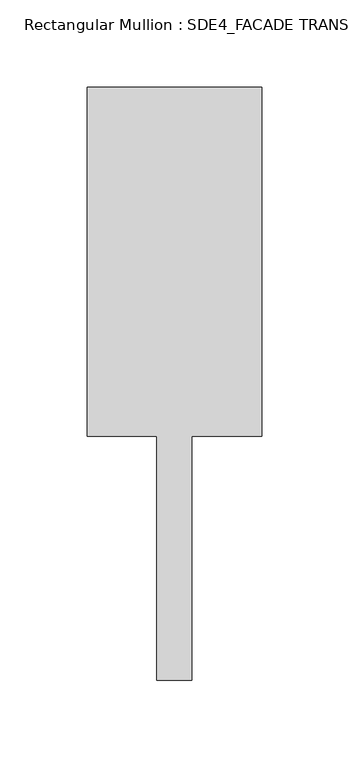
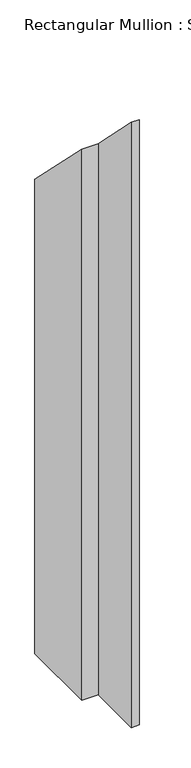
"""IFC4 building model written with IfcOpenShell, lengths in millimetres: member geometry, Rectangular Mullion : SDE4_FACADE TRANSOM TYPE 1."""

from ifc_helpers import new_model, si_unit, origin, place, context, project, spatial, faceted_brep, source, transform, mapped, element, save


def rectangular_mullion_sde4_facade_transom_type_1_15dbdb44(model_context):
    return source(origin(), model_context, "Body", "Brep", [
        faceted_brep([(50.0, 132.5, -1362.8200128), (50.0, -67.5, -1362.8200128), (10.0, -67.5, -1362.8200128), (10.0, -207.5, -1362.8200128), (-10.0, -207.5, -1362.8200128), (-10.0, -67.5, -1362.8200128), (-50.0, -67.5, -1362.8200128), (-50.0, 132.5, -1362.8200128), (-50.0, 132.5, -132.5), (50.0, 132.5, -132.5), (-50.0, -67.5, 67.5), (-10.0, -67.5, 67.5), (-10.0, -207.5, 207.5), (10.0, -207.5, 207.5), (10.0, -67.5, 67.5), (50.0, -67.5, 67.5)], [[[0, 1, 2, 3, 4, 5, 6, 7]], [[8, 9, 0, 7]], [[10, 8, 7, 6]], [[11, 10, 6, 5]], [[12, 11, 5, 4]], [[13, 12, 4, 3]], [[14, 13, 3, 2]], [[15, 14, 2, 1]], [[9, 15, 1, 0]], [[9, 8, 10, 11, 12, 13, 14, 15]]]),
    ])


if __name__ == "__main__":
    model = new_model("IFC4")
    model_context = context("Model", 3, world=origin())
    ifc_project = project(units=[si_unit("LENGTHUNIT", "METRE", prefix="MILLI")], contexts=[model_context])
    site = spatial("IfcSite", under=ifc_project)
    building = spatial("IfcBuilding", under=site)
    placement = place(None, origin())
    rectangular_mullion_sde4_facade_transom_type_1_shape = rectangular_mullion_sde4_facade_transom_type_1_15dbdb44(model_context)
    element("IfcMember", 1, ObjectType="Rectangular Mullion : SDE4_FACADE TRANSOM TYPE 1", at=placement, inside=building, context=model_context, shape_type="MappedRepresentation", body=[
        mapped(rectangular_mullion_sde4_facade_transom_type_1_shape, transform((0.0, 0.0, 0.0), x_axis=(1.0, 0.0, 0.0), y_axis=(0.0, 1.0, 0.0), z_axis=(0.0, 0.0, 1.0))),
    ])
    save(model, "model.ifc")

# Revit data of these elements
# Type "Rectangular Mullion : SDE4_FACADE TRANSOM TYPE 1"
#   built-in parameter 1007322 = 1.11549 (stored number, unit not read)
#   built-in parameter 1007321 = 0.164042 (stored number, unit not read)
#   built-in parameter 1007320 = 0.164042 (stored number, unit not read)
